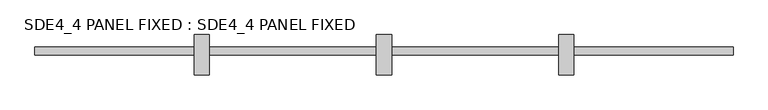
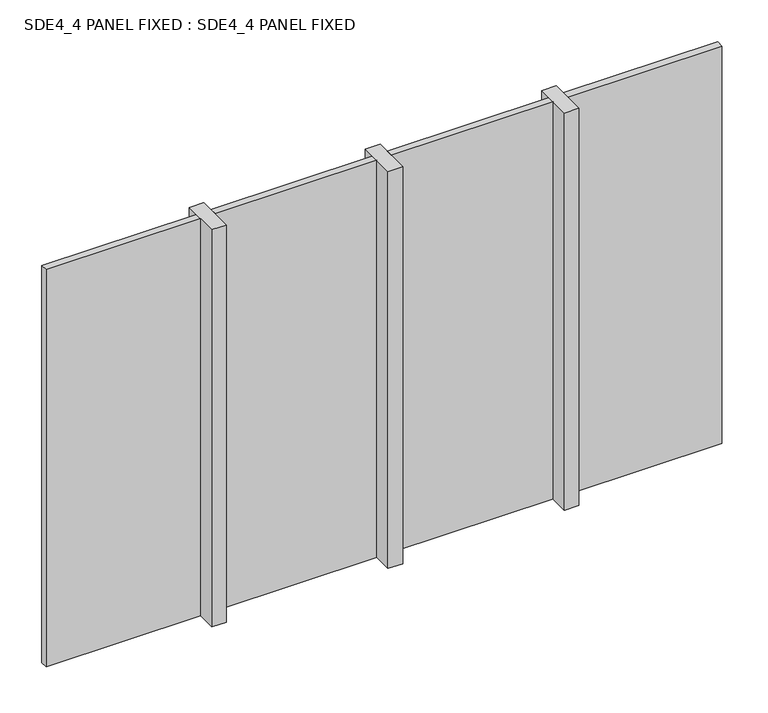
"""IFC4 building model written with IfcOpenShell, lengths in millimetres: plate geometry, SDE4_4 PANEL FIXED : SDE4_4 PANEL FIXED."""

from ifc_helpers import new_model, si_unit, origin, origin_with_axes, place, context, project, spatial, polyline, outline, extrude, source, transform, mapped, element, save


def sde4_4_panel_fixed_sde4_4_panel_fixed_bb660ca6(model_context):
    return source(origin(), model_context, "Body", "SweptSolid", [
        extrude(outline(polyline([(-1150.0, 132.5), (-1150.0, -132.5), (-1250.0, -132.5), (-1250.0, 132.5), (-1150.0, 132.5)])), origin_with_axes(), (0.0, 0.0, 1.0), 2860.0),
        extrude(outline(polyline([(50.0, 132.5), (50.0, -132.5), (-50.0, -132.5), (-50.0, 132.5), (50.0, 132.5)])), origin_with_axes(), (0.0, 0.0, 1.0), 2860.0),
        extrude(outline(polyline([(1250.0, 132.5), (1250.0, -132.5), (1150.0, -132.5), (1150.0, 132.5), (1250.0, 132.5)])), origin_with_axes(), (0.0, 0.0, 1.0), 2860.0),
        extrude(outline(polyline([(2299.0, 50.0), (2299.0, 0.0), (1250.0, 0.0), (1250.0, 50.0), (2299.0, 50.0)])), origin_with_axes(), (0.0, 0.0, 1.0), 2860.0),
        extrude(outline(polyline([(1150.0, 50.0), (1150.0, 0.0), (50.0, 0.0), (50.0, 50.0), (1150.0, 50.0)])), origin_with_axes(), (0.0, 0.0, 1.0), 2860.0),
        extrude(outline(polyline([(-50.0, 50.0), (-50.0, 0.0), (-1150.0, 0.0), (-1150.0, 50.0), (-50.0, 50.0)])), origin_with_axes(), (0.0, 0.0, 1.0), 2860.0),
        extrude(outline(polyline([(-1250.0, 50.0), (-1250.0, 0.0), (-2300.0, 0.0), (-2300.0, 50.0), (-1250.0, 50.0)])), origin_with_axes(), (0.0, 0.0, 1.0), 2860.0),
    ])


if __name__ == "__main__":
    model = new_model("IFC4")
    model_context = context("Model", 3, world=origin())
    ifc_project = project(units=[si_unit("LENGTHUNIT", "METRE", prefix="MILLI")], contexts=[model_context])
    site = spatial("IfcSite", under=ifc_project)
    building = spatial("IfcBuilding", under=site)
    placement = place(None, origin())
    sde4_4_panel_fixed_sde4_4_panel_fixed_shape = sde4_4_panel_fixed_sde4_4_panel_fixed_bb660ca6(model_context)
    element("IfcPlate", 1, ObjectType="SDE4_4 PANEL FIXED : SDE4_4 PANEL FIXED", at=placement, inside=building, context=model_context, shape_type="MappedRepresentation", body=[
        mapped(sde4_4_panel_fixed_sde4_4_panel_fixed_shape, transform((0.0, 0.0, 0.0), x_axis=(1.0, 0.0, 0.0), y_axis=(0.0, 1.0, 0.0), z_axis=(0.0, 0.0, 1.0))),
    ])
    save(model, "model.ifc")

# Revit data of these elements
# Type "SDE4_4 PANEL FIXED : SDE4_4 PANEL FIXED"
#   Type Mark = "CW-GLASS"
#   Analytic Construction = "<None>"
#   Glass = Glass
#   Frame = Aluminium
# Element 1 (IfcPlate, "SDE4_4 PANEL FIXED : SDE4_4 PANEL FIXED")
#   Materials on its faces: "Glass", "Aluminium"
# Materials
#   "Glass": class "Glass", colour RGB 0 128 192, transparency 0.9, Keynote = "L40", Cost = 0
#   "Aluminium": class "Unassigned", colour RGB 247 247 247, transparency 0, Cost = 0
